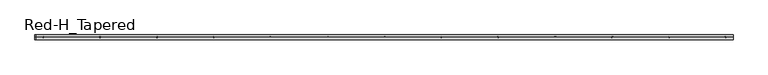
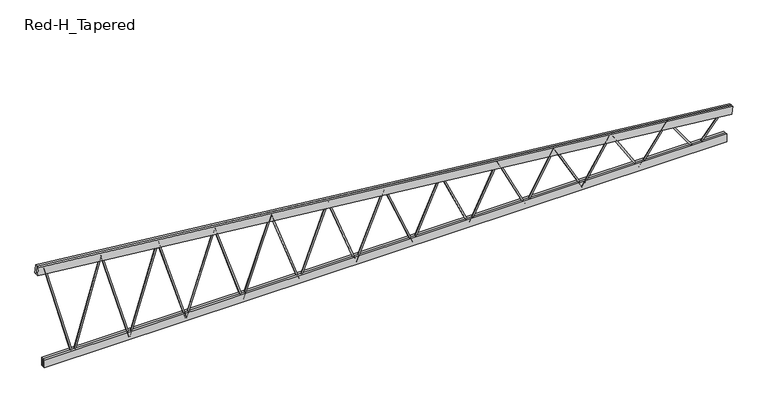
"""IFC4 building model written with IfcOpenShell, lengths in millimetres: beam geometry, Construction_Frames_RedBuilt_Openweb_Red-H_Tapered : Red-H_Tapered."""

from ifc_helpers import new_model, si_unit, point, frame, origin, origin_2d, place, context, project, spatial, polyline, circle_curve, trimmed, segment, composite_curve, outline, extrude, source, transform, mapped, element, save


def red_h_tapered_f993d055(model_context):
    return source(origin(), model_context, "Body", "SweptSolid", [
        extrude(outline(composite_curve([segment(trimmed(circle_curve(origin_2d(), 12.7), [point((0.0, -12.7))], [point((0.0, 12.7))], False, "CARTESIAN"), True, "CONTINUOUS"), segment(trimmed(circle_curve(origin_2d(), 12.7), [point((0.0, 12.7))], [point((0.0, -12.7))], False, "CARTESIAN"), True, "CONTINUOUS")], self_intersect=False)), frame((-491.6619792, 0.0, -367.0101562), z_axis=(-0.3587068924496881, 0.0, 0.9334502479024193), x_axis=(0.0, -1.0, 0.0)), (0.0, 0.0, 1.0), 1370.6510511),
        extrude(outline(composite_curve([segment(trimmed(circle_curve(origin_2d(), 12.7), [point((0.0, 12.7))], [point((0.0, -12.6999999))], False, "CARTESIAN"), True, "CONTINUOUS"), segment(trimmed(circle_curve(origin_2d(), 12.7), [point((0.0, -12.6999999))], [point((0.0, 12.7))], False, "CARTESIAN"), True, "CONTINUOUS")], self_intersect=False)), frame((-1474.9859375, 0.0, -367.0101562), z_axis=(0.35870689244968823, 0.0, 0.9334502479024192), x_axis=(0.0, -1.0, 0.0)), (0.0, 0.0, 1.0), 1370.6510511),
        extrude(outline(composite_curve([segment(trimmed(circle_curve(origin_2d(), 12.7), [point((0.0, -12.7))], [point((0.0, 12.7))], False, "CARTESIAN"), True, "CONTINUOUS"), segment(trimmed(circle_curve(origin_2d(), 12.7), [point((0.0, 12.7))], [point((0.0, -12.7))], False, "CARTESIAN"), True, "CONTINUOUS")], self_intersect=False)), frame((-1474.9859375, 0.0, -367.0101562), z_axis=(-0.33588189777741245, 0.0, 0.941904109103174), x_axis=(0.0, -1.0, 0.0)), (0.0, 0.0, 1.0), 1463.7942158),
        extrude(outline(composite_curve([segment(trimmed(circle_curve(origin_2d(), 12.7), [point((0.0, -12.7))], [point((0.0, 12.7))], False, "CARTESIAN"), True, "CONTINUOUS"), segment(trimmed(circle_curve(origin_2d(), 12.7), [point((0.0, 12.7))], [point((0.0, -12.7))], False, "CARTESIAN"), True, "CONTINUOUS")], self_intersect=False)), frame((-2458.3098958, 0.0, -367.0101562), z_axis=(0.3358818977774164, 0.0, 0.9419041091031726), x_axis=(0.0, -1.0, 0.0)), (0.0, 0.0, 1.0), 1463.7942158),
        extrude(outline(composite_curve([segment(trimmed(circle_curve(origin_2d(), 12.7), [point((0.0, 12.7))], [point((0.0, -12.7000001))], False, "CARTESIAN"), True, "CONTINUOUS"), segment(trimmed(circle_curve(origin_2d(), 12.7), [point((0.0, -12.7000001))], [point((0.0, 12.7))], False, "CARTESIAN"), True, "CONTINUOUS")], self_intersect=False)), frame((-2458.3098958, 0.0, -367.0101562), z_axis=(-0.31563315978368506, 0.0, 0.9488812931262619), x_axis=(0.0, -1.0, 0.0)), (0.0, 0.0, 1.0), 1557.7006532),
        extrude(outline(composite_curve([segment(trimmed(circle_curve(origin_2d(), 12.7), [point((0.0, -12.7))], [point((0.0, 12.7000001))], False, "CARTESIAN"), True, "CONTINUOUS"), segment(trimmed(circle_curve(origin_2d(), 12.7), [point((0.0, 12.7000001))], [point((0.0, -12.7))], False, "CARTESIAN"), True, "CONTINUOUS")], self_intersect=False)), frame((-3441.6338542, 0.0, -367.0101562), z_axis=(0.3156331597836845, 0.0, 0.948881293126262), x_axis=(0.0, -1.0, 0.0)), (0.0, 0.0, 1.0), 1557.7006532),
        extrude(outline(composite_curve([segment(trimmed(circle_curve(origin_2d(), 12.7), [point((0.0, 12.7))], [point((0.0, -12.7))], False, "CARTESIAN"), True, "CONTINUOUS"), segment(trimmed(circle_curve(origin_2d(), 12.7), [point((0.0, -12.7))], [point((0.0, 12.7))], False, "CARTESIAN"), True, "CONTINUOUS")], self_intersect=False)), frame((-3441.6338542, 0.0, -367.0101562), z_axis=(-0.29757293874902985, 0.0, 0.9546990866887148), x_axis=(0.0, -1.0, 0.0)), (0.0, 0.0, 1.0), 1652.2402246),
        extrude(outline(composite_curve([segment(trimmed(circle_curve(origin_2d(), 12.7), [point((0.0, -12.7))], [point((0.0, 12.7))], False, "CARTESIAN"), True, "CONTINUOUS"), segment(trimmed(circle_curve(origin_2d(), 12.7), [point((0.0, 12.7))], [point((0.0, -12.7))], False, "CARTESIAN"), True, "CONTINUOUS")], self_intersect=False)), frame((-4424.9578125, 0.0, -367.0101562), z_axis=(0.2975729387490355, 0.0, 0.9546990866887131), x_axis=(0.0, -1.0, 0.0)), (0.0, 0.0, 1.0), 1652.2402246),
        extrude(outline(composite_curve([segment(trimmed(circle_curve(origin_2d(), 12.7), [point((0.0, 12.7))], [point((0.0, -12.7))], False, "CARTESIAN"), True, "CONTINUOUS"), segment(trimmed(circle_curve(origin_2d(), 12.7), [point((0.0, -12.7))], [point((0.0, 12.7))], False, "CARTESIAN"), True, "CONTINUOUS")], self_intersect=False)), frame((-4424.9578125, 0.0, -367.0101562), z_axis=(-0.281382200562923, 0.0, 0.9595957780265434), x_axis=(0.0, -1.0, 0.0)), (0.0, 0.0, 1.0), 1747.3101645),
        extrude(outline(composite_curve([segment(trimmed(circle_curve(origin_2d(), 12.7), [point((0.0, -12.7))], [point((0.0, 12.6999999))], False, "CARTESIAN"), True, "CONTINUOUS"), segment(trimmed(circle_curve(origin_2d(), 12.7), [point((0.0, 12.6999999))], [point((0.0, -12.7))], False, "CARTESIAN"), True, "CONTINUOUS")], self_intersect=False)), frame((-5408.2817708, 0.0, -367.0101562), z_axis=(0.28138220056292157, 0.0, 0.9595957780265438), x_axis=(0.0, -1.0, 0.0)), (0.0, 0.0, 1.0), 1747.3101645),
        extrude(outline(composite_curve([segment(trimmed(circle_curve(origin_2d(), 12.7), [point((0.0, 12.7))], [point((0.0, -12.7))], False, "CARTESIAN"), True, "CONTINUOUS"), segment(trimmed(circle_curve(origin_2d(), 12.7), [point((0.0, -12.7))], [point((0.0, 12.7))], False, "CARTESIAN"), True, "CONTINUOUS")], self_intersect=False)), frame((-5408.2817708, 0.0, -367.0101562), z_axis=(-0.2667974845482189, 0.0, 0.9637526146469035), x_axis=(0.0, -1.0, 0.0)), (0.0, 0.0, 1.0), 1842.828391),
        extrude(outline(composite_curve([segment(trimmed(circle_curve(origin_2d(), 12.7), [point((0.0, 12.7000001))], [point((0.0, -12.6999999))], False, "CARTESIAN"), True, "CONTINUOUS"), segment(trimmed(circle_curve(origin_2d(), 12.7), [point((0.0, -12.6999999))], [point((0.0, 12.7000001))], False, "CARTESIAN"), True, "CONTINUOUS")], self_intersect=False)), frame((5408.2817708, 0.0, -367.0101562), z_axis=(0.6439089672678225, 0.0, 0.7651021120556957), x_axis=(0.0, -1.0, 0.0)), (0.0, 0.0, 1.0), 763.5582111),
        extrude(outline(composite_curve([segment(trimmed(circle_curve(origin_2d(), 12.7), [point((0.0, -12.7))], [point((0.0, 12.7))], False, "CARTESIAN"), True, "CONTINUOUS"), segment(trimmed(circle_curve(origin_2d(), 12.7), [point((0.0, 12.7))], [point((0.0, -12.7))], False, "CARTESIAN"), True, "CONTINUOUS")], self_intersect=False)), frame((5408.2817708, 0.0, -367.0101562), z_axis=(-0.5839355800775429, 0.0, 0.8117999989649566), x_axis=(0.0, -1.0, 0.0)), (0.0, 0.0, 1.0), 841.9798278),
        extrude(outline(composite_curve([segment(trimmed(circle_curve(origin_2d(), 12.7), [point((0.0, 12.7))], [point((0.0, -12.7))], False, "CARTESIAN"), True, "CONTINUOUS"), segment(trimmed(circle_curve(origin_2d(), 12.7), [point((0.0, -12.7))], [point((0.0, 12.7))], False, "CARTESIAN"), True, "CONTINUOUS")], self_intersect=False)), frame((4424.9578125, 0.0, -367.0101562), z_axis=(0.5839355800775407, 0.0, 0.8117999989649581), x_axis=(0.0, -1.0, 0.0)), (0.0, 0.0, 1.0), 841.9798278),
        extrude(outline(composite_curve([segment(trimmed(circle_curve(origin_2d(), 12.7), [point((0.0, -12.7000001))], [point((0.0, 12.7))], False, "CARTESIAN"), True, "CONTINUOUS"), segment(trimmed(circle_curve(origin_2d(), 12.7), [point((0.0, 12.7))], [point((0.0, -12.7000001))], False, "CARTESIAN"), True, "CONTINUOUS")], self_intersect=False)), frame((4424.9578125, 0.0, -367.0101562), z_axis=(-0.531855224790945, 0.0, 0.8468352967741563), x_axis=(0.0, -1.0, 0.0)), (0.0, 0.0, 1.0), 924.4282208),
        extrude(outline(composite_curve([segment(trimmed(circle_curve(origin_2d(), 12.7), [point((0.0, 12.7))], [point((0.0, -12.7))], False, "CARTESIAN"), True, "CONTINUOUS"), segment(trimmed(circle_curve(origin_2d(), 12.7), [point((0.0, -12.7))], [point((0.0, 12.7))], False, "CARTESIAN"), True, "CONTINUOUS")], self_intersect=False)), frame((3441.6338542, 0.0, -367.0101562), z_axis=(0.5318552247909429, 0.0, 0.8468352967741576), x_axis=(0.0, -1.0, 0.0)), (0.0, 0.0, 1.0), 924.4282208),
        extrude(outline(composite_curve([segment(trimmed(circle_curve(origin_2d(), 12.7), [point((0.0, -12.7000001))], [point((0.0, 12.7))], False, "CARTESIAN"), True, "CONTINUOUS"), segment(trimmed(circle_curve(origin_2d(), 12.7), [point((0.0, 12.7))], [point((0.0, -12.7000001))], False, "CARTESIAN"), True, "CONTINUOUS")], self_intersect=False)), frame((3441.6338542, 0.0, -367.0101562), z_axis=(-0.4868337333664658, 0.0, 0.8734946571424859), x_axis=(0.0, -1.0, 0.0)), (0.0, 0.0, 1.0), 1009.9176484),
        extrude(outline(composite_curve([segment(trimmed(circle_curve(origin_2d(), 12.7), [point((0.0, 12.7000001))], [point((0.0, -12.7))], False, "CARTESIAN"), True, "CONTINUOUS"), segment(trimmed(circle_curve(origin_2d(), 12.7), [point((0.0, -12.7))], [point((0.0, 12.7000001))], False, "CARTESIAN"), True, "CONTINUOUS")], self_intersect=False)), frame((2458.3098958, 0.0, -367.0101562), z_axis=(0.4868337333664665, 0.0, 0.8734946571424854), x_axis=(0.0, -1.0, 0.0)), (0.0, 0.0, 1.0), 1009.9176484),
        extrude(outline(composite_curve([segment(trimmed(circle_curve(origin_2d(), 12.7), [point((0.0, -12.7))], [point((0.0, 12.7))], False, "CARTESIAN"), True, "CONTINUOUS"), segment(trimmed(circle_curve(origin_2d(), 12.7), [point((0.0, 12.7))], [point((0.0, -12.7))], False, "CARTESIAN"), True, "CONTINUOUS")], self_intersect=False)), frame((2458.3098958, 0.0, -367.0101562), z_axis=(-0.4478865129810261, 0.0, 0.8940904157241018), x_axis=(0.0, -1.0, 0.0)), (0.0, 0.0, 1.0), 1097.737853),
        extrude(outline(composite_curve([segment(trimmed(circle_curve(origin_2d(), 12.7), [point((0.0, 12.7000001))], [point((0.0, -12.7))], False, "CARTESIAN"), True, "CONTINUOUS"), segment(trimmed(circle_curve(origin_2d(), 12.7), [point((0.0, -12.7))], [point((0.0, 12.7000001))], False, "CARTESIAN"), True, "CONTINUOUS")], self_intersect=False)), frame((1474.9859375, 0.0, -367.0101562), z_axis=(0.44788651298103027, 0.0, 0.8940904157240998), x_axis=(0.0, -1.0, 0.0)), (0.0, 0.0, 1.0), 1097.737853),
        extrude(outline(composite_curve([segment(trimmed(circle_curve(origin_2d(), 12.7), [point((0.0, -12.7))], [point((0.0, 12.6999999))], False, "CARTESIAN"), True, "CONTINUOUS"), segment(trimmed(circle_curve(origin_2d(), 12.7), [point((0.0, 12.6999999))], [point((0.0, -12.7))], False, "CARTESIAN"), True, "CONTINUOUS")], self_intersect=False)), frame((1474.9859375, 0.0, -367.0101562), z_axis=(-0.41407584953051496, 0.0, 0.9102423802677957), x_axis=(0.0, -1.0, 0.0)), (0.0, 0.0, 1.0), 1187.3717816),
        extrude(outline(composite_curve([segment(trimmed(circle_curve(origin_2d(), 12.7), [point((0.0, 12.7))], [point((0.0, -12.7))], False, "CARTESIAN"), True, "CONTINUOUS"), segment(trimmed(circle_curve(origin_2d(), 12.7), [point((0.0, -12.7))], [point((0.0, 12.7))], False, "CARTESIAN"), True, "CONTINUOUS")], self_intersect=False)), frame((491.6619792, 0.0, -367.0101562), z_axis=(0.4140758495305158, 0.0, 0.9102423802677954), x_axis=(0.0, -1.0, 0.0)), (0.0, 0.0, 1.0), 1187.3717816),
        extrude(outline(composite_curve([segment(trimmed(circle_curve(origin_2d(), 12.7), [point((0.0, -12.7000001))], [point((0.0, 12.7))], False, "CARTESIAN"), True, "CONTINUOUS"), segment(trimmed(circle_curve(origin_2d(), 12.7), [point((0.0, 12.7))], [point((0.0, -12.7000001))], False, "CARTESIAN"), True, "CONTINUOUS")], self_intersect=False)), frame((491.6619792, 0.0, -367.0101562), z_axis=(-0.38458022954457244, 0.0, 0.9230915702374517), x_axis=(0.0, -1.0, 0.0)), (0.0, 0.0, 1.0), 1278.4379991),
        extrude(outline(composite_curve([segment(trimmed(circle_curve(origin_2d(), 12.7), [point((0.0, 12.7000001))], [point((0.0, -12.7))], False, "CARTESIAN"), True, "CONTINUOUS"), segment(trimmed(circle_curve(origin_2d(), 12.7), [point((0.0, -12.7))], [point((0.0, 12.7000001))], False, "CARTESIAN"), True, "CONTINUOUS")], self_intersect=False)), frame((-491.6619792, 0.0, -367.0101562), z_axis=(0.38458022954454074, 0.0, 0.9230915702374648), x_axis=(0.0, -1.0, 0.0)), (0.0, 0.0, 1.0), 1278.4379991),
        extrude(outline(polyline([(-5925.34375, -41.275), (-5925.34375, -3.175), (5925.34375, -3.175), (5925.34375, -41.275), (-5925.34375, -41.275)])), frame((0.0, 0.0, -386.0601562), z_axis=(0.0, 0.0, 1.0), x_axis=(1.0, 0.0, 0.0)), (0.0, 0.0, 1.0), 139.7),
        extrude(outline(polyline([(-5925.34375, 3.175), (-5925.34375, 41.275), (5925.34375, 41.275), (5925.34375, 3.175), (-5925.34375, 3.175)])), frame((0.0, 0.0, -386.0601562), z_axis=(0.0, 0.0, 1.0), x_axis=(1.0, 0.0, 0.0)), (0.0, 0.0, 1.0), 139.7),
        extrude(outline(polyline([(0.0, -38.1), (0.0, 0.0), (12119.7774574, 0.0), (12119.7774574, -38.1), (0.0, -38.1)])), frame((-6041.4910576, -3.175, 1346.6618319), z_axis=(0.10413248134608866, 0.0, 0.9945634350450988), x_axis=(0.9945634350450988, 0.0, -0.10413248134608866)), (0.0, 0.0, 1.0), 139.7),
        extrude(outline(polyline([(0.0, -38.1), (0.0, 0.0), (12119.7774574, 0.0), (12119.7774574, -38.1), (0.0, -38.1)])), frame((-6041.4910576, 41.275, 1346.6618319), z_axis=(0.10413248134608866, 0.0, 0.9945634350450988), x_axis=(0.9945634350450988, 0.0, -0.10413248134608866)), (0.0, 0.0, 1.0), 139.7),
    ])


if __name__ == "__main__":
    model = new_model("IFC4")
    model_context = context("Model", 3, world=origin())
    ifc_project = project(units=[si_unit("LENGTHUNIT", "METRE", prefix="MILLI")], contexts=[model_context])
    site = spatial("IfcSite", under=ifc_project)
    building = spatial("IfcBuilding", under=site)
    placement = place(None, origin())
    red_h_tapered_shape = red_h_tapered_f993d055(model_context)
    element("IfcBeam", 1, ObjectType="Construction_Frames_RedBuilt_Openweb_Red-H_Tapered : Red-H_Tapered", at=placement, inside=building, context=model_context, shape_type="MappedRepresentation", body=[
        mapped(red_h_tapered_shape, transform((0.0, 0.0, 0.0), x_axis=(1.0, 0.0, 0.0), y_axis=(0.0, 1.0, 0.0), z_axis=(0.0, 0.0, 1.0))),
    ])
    save(model, "model.ifc")

# Revit data of these elements
# Type "Construction_Frames_RedBuilt_Openweb_Red-H_Tapered : Red-H_Tapered"
#   Youtube clip = ""
#   Weight Net (Kg) = "0"
#   Webs = "Up to 2\" diameter tubular steel"
#   Uniformat II Description = ""
#   Uniformat II Code = ""
#   Uniclass 2015 Name = "Softwood trusses"
#   Uniclass 2015 Code = "Pr_20_85_90_81"
#   Uniclass 2.0 Description = "Structural Framing Systems"
#   Uniclass 2.0 Code = "SS-15-10-75"
#   Uniclass 1.4 Description = "Trusses"
#   Uniclass 1.4 Code = "L3523"
#   UNSPSC Code = "30103606"
#   Technical description = "http://www.redbuilt.com/reference/literature-and-other-resources"
#   Region South America = "None"
#   Region Oceania = "None"
#   Region North America = "US"
#   Region Middle East = "None"
#   Region Europe = "None"
#   Region Asia = "None"
#   Region Antarctica = "None"
#   Region Africa = "None"
#   QR code = "http://bimobject.com/redbuilt/product/redbuilt-0003"
#   Product url = "http://www.redbuilt.com/products/default.aspx?id=2"
#   Product group = "Wood Trusses"
#   Product family = "Construction"
#   Product data url = "https://bimobject.com/redbuilt/product/redbuilt-0003"
#   Product certification = ""
#   Product SKU = "redbuilt-0003"
#   Product Page URL = "http://www.redbuilt.com/commercial-systems/red-m-red-h-open-web-trusses"
#   Product Guid = "2c5793f2-6ffb-4665-b825-cf90c048e711"
#   Product Documentation Link = "http://www.redbuilt.com/documents/OW_Guide_2017_07_LowRes_wLinks.pdf"
#   OmniClass Description = "Wood Trusses"
#   OmniClass Code = "23-13 35 19 13 17"
#   NBS Reference Description = ""
#   NBS Reference Code = ""
#   Material secondary = "Steel"
#   Material main = "Wood"
#   Masterformat 2014 Description = "Metal-Web Wood Joists"
#   Masterformat 2014 Code = "06 17 36"
#   Manufacturer name = "RedBuilt"
#   Manufacturer country = "United States"
#   Installation instructions = "http://www.redbuilt.com/documents/Installation_Sheets_Open-Web.pdf"
#   IFC Classification = ""
#   EAN code = ""
#   Design country = "United States"
#   Product Information = "http://redbuilt.com/products/default.aspx?id=2"
#   Model = "Red-H-Tapered"
#   Manufacturer URL = "http://redbuilt.com/"
#   Manufacturer = "RedBuilt™"
#   Description = "Open Web Truss"
#   Date of publishing = "8/17/2010"
#   Contact us = "http://redbuilt.com/contact/"
#   Chords = "Double 1½\" x 5½\" MSR lumber"
#   COBIe Type Category = ""
#   Brand url = "http://www.redbuilt.com"
#   BIMobject main category code = "construction"
#   BIMobject main category = "Construction"
#   BIMobject category code = "construction-frames-trusses"
#   BIMobject category = "Frames & Trusses"
#   Web Radius = 0' - 0 1/2"
#   Web Layout Offset Start [instance default] = 0' - 5"
#   Web Layout Offset End [instance default] = 0' - 5"
#   Web Diameter = 0' - 1"
#   TotalLength [instance default] = 20' - 0"
#   Span Minimum = 4' - 0"
#   Span Maximum = 70' - 0"
#   Span Limit [instance default] = 20' - 0"
#   Nominal width = 0' - 0"
#   Nominal height = 0' - 0"
#   Inner Depth Top [instance default] = 0' - 2.76372"
#   Depth Start [instance default] = 6' - 0"
#   Top Chord Length [instance default] = 20' - 1.19701"
#   TC Extension Start Aux [instance default] = 0' - 0"
#   TC Extension End Aux [instance default] = 0' - 0"
#   T-B Chord Length Difference L [instance default] = 0' - 4"
#   T-B Chord Length Difference [instance default] = 0' - 4"
#   Height 2 [instance default] = 6' - 0"
#   Depth Minimum at Wall = 2' - 0"
#   Depth Maximum at Wall = 6' - 0"
#   Depth Lower End [instance default] = 2' - 0"
#   Depth Higher End [instance default] = 6' - 0"
#   Depth End [instance default] = 2' - 0"
#   Depth 2 [instance default] = 2' - 0"
#   Chord Width = 0' - 3 1/4"
#   Chord Thickness = 0' - 1 1/2"
#   Chord Depth = 0' - 5 1/2"
#   Offset Start [instance default] = 0' - 0"
#   TC Extension Start [instance default] = 0' - 0"
#   End Panel = 0' - 5"
#   Offset End [instance default] = 0' - 0"
#   TC Extension End [instance default] = 0' - 0"
#   Length [instance default] = 20' - 0"
#   Angle [instance default] = 5.71059°
#   Span Limit Warning [instance default] = no
#   Edition number = 1
#   Top Bearing Start [instance default] = yes
#   Top Bearing End [instance default] = yes
#   Bottom Bearing Start [instance default] = no
#   Bottom Bearing End [instance default] = no
#   8 Panels [instance default] = yes
#   16 Panels [instance default] = no
#   12 Panels [instance default] = no
#   Web Material = RedBuilt-Steel, Galvanized
#   Clip Material = RedBuilt-Steel, Galvanized
#   Chords Material = RedBuilt-MSR
#   URL = ""
#   Assembly Code = ""
# Element 1 (IfcBeam, "Construction_Frames_RedBuilt_Openweb_Red-H_Tapered : Red-H_Tapered")
#   TotalLength = 39' - 6 9/16"
#   Span Limit = 39' - 6 9/16"
#   Inner Depth Top = 0' - 2.76503"
#   Top Chord Length = 39' - 9.15659"
#   Depth 2 = 4' - 1 11/16"
#   Angle = 5.97719°
#   8 Panels = no
#   12 Panels = yes
#   Materials on its faces: "RedBuilt-Steel, Galvanized", "RedBuilt-MSR"
# Materials
#   "RedBuilt-Steel, Galvanized": class "Metal", colour RGB 164 172 176, transparency 0, Manufacturer = "RedBuilt. LLC", Comments = "Openweb Metal Web", URL = "http://www.redbuilt.com/", Description = "Galvanized steel", Cost = 0
#   "RedBuilt-MSR": class "Wood", colour RGB 213 182 136, transparency 0, Manufacturer = "RedBuilt, LLC", URL = "http://www.redbuilt.com/", Cost = 0
